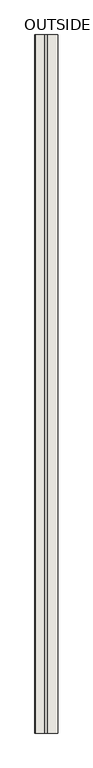
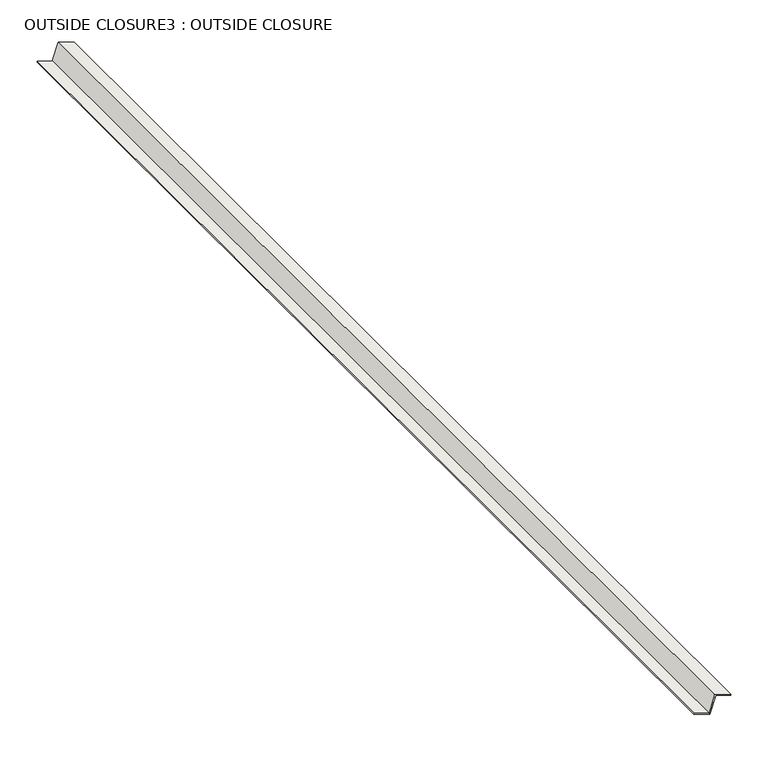
"""IFC4 building model written with IfcOpenShell, lengths in millimetres: wall geometry, OUTSIDE CLOSURE3 : OUTSIDE CLOSURE."""

from ifc_helpers import new_model, si_unit, frame, origin, place, context, project, spatial, polyline, outline, extrude, source, transform, mapped, element, save


def outside_closure3_outside_closure_23ee7d9d(model_context):
    return source(origin(), model_context, "Body", "SweptSolid", [
        extrude(outline(polyline([(5859.8565193, 21567.9997107), (5868.1723106, 21543.1610281), (5841.0628524, 21534.0849995), (5848.8746563, 21510.7516916), (5847.3430053, 21510.2389071), (5839.0272141, 21535.0775898), (5866.1629485, 21544.1624155), (5858.3511446, 21567.4957234), (5859.8565193, 21567.9997107)])), frame((0.0, -2319.6634634, 0.0), z_axis=(0.0, 1.0, 0.0), x_axis=(0.0, 0.0, 1.0)), (0.0, 0.0, 1.0), 1767.3456389),
    ])


if __name__ == "__main__":
    model = new_model("IFC4")
    model_context = context("Model", 3, world=origin())
    ifc_project = project(units=[si_unit("LENGTHUNIT", "METRE", prefix="MILLI")], contexts=[model_context])
    site = spatial("IfcSite", under=ifc_project)
    building = spatial("IfcBuilding", under=site)
    placement = place(None, origin())
    outside_closure3_outside_closure_shape = outside_closure3_outside_closure_23ee7d9d(model_context)
    element("IfcWall", 1, ObjectType="OUTSIDE CLOSURE3 : OUTSIDE CLOSURE", at=placement, inside=building, context=model_context, shape_type="MappedRepresentation", body=[
        mapped(outside_closure3_outside_closure_shape, transform((0.0, 0.0, 0.0), x_axis=(1.0, 0.0, 0.0), y_axis=(0.0, 1.0, 0.0), z_axis=(0.0, 0.0, 1.0))),
    ])
    save(model, "model.ifc")

# Revit data of these elements
# Element 1 (IfcWall, "OUTSIDE CLOSURE3 : OUTSIDE CLOSURE")
#   Materials on its faces: "OUTSIDE CLOSURE"
# Materials
#   "OUTSIDE CLOSURE": class "Metal", colour RGB 247 247 247, transparency 0, Cost = 0
